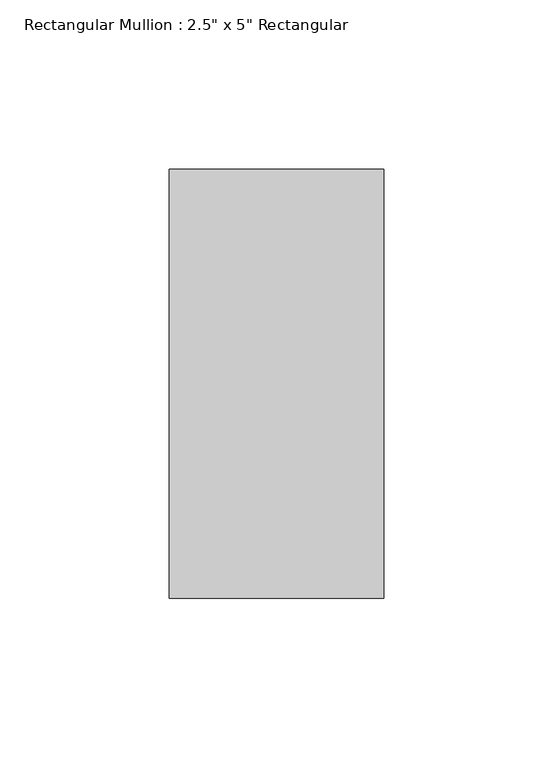
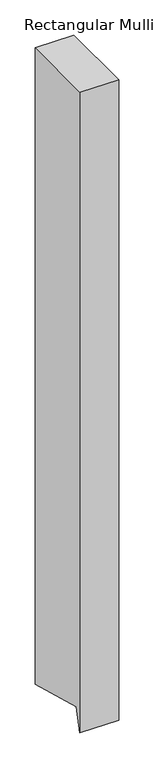
"""IFC4 building model written with IfcOpenShell, lengths in millimetres: member geometry."""

import ifcopenshell
import ifcopenshell.guid

model = None  # the IFC model being written
_history = None  # IfcOwnerHistory: only IFC2X3 demands one
_inside = {}  # id of a spatial element -> (the spatial element, [elements in it])
_under = {}  # id of a project, library or spatial element -> (it, [spatial elements below it])
_declared = {}  # id of a project -> (the project, [libraries it declares])
_typed = {}  # id of a type object -> (the type object, [elements of that type])
_made_of = {}  # id of a material, layer set ... -> (it, [elements and type objects made of it])


def new_model(schema):
    """Start an empty IFC model of exactly this schema.

    Asked for "IFC4X3", IfcOpenShell would pick the latest addendum, in which some entities
    have other attributes; the version numbers below select the first issue.
    IFC2X3 requires an IfcOwnerHistory on every rooted entity: one is made here for all.
    """
    global model, _history
    if schema == "IFC4X3":
        model = ifcopenshell.file(schema_version=(4, 3, 0, 0))
    else:
        model = ifcopenshell.file(schema=schema)
    _inside.clear()
    _under.clear()
    _declared.clear()
    _typed.clear()
    _made_of.clear()
    _history = None
    if model.schema == "IFC2X3":
        org = make("IfcOrganization", Name="unknown")
        user = make(
            "IfcPersonAndOrganization",
            ThePerson=make("IfcPerson", FamilyName="unknown"),
            TheOrganization=org,
        )
        app = make(
            "IfcApplication",
            ApplicationDeveloper=org,
            Version="unknown",
            ApplicationFullName="unknown",
            ApplicationIdentifier="unknown",
        )
        _history = make(
            "IfcOwnerHistory",
            OwningUser=user,
            OwningApplication=app,
            ChangeAction="ADDED",
            CreationDate=0,
        )
    return model


def make(cls, **values):
    """One entity of the class cls with the attributes given. An attribute that is None is left unset."""
    return model.create_entity(
        cls, **{name: value for name, value in values.items() if value is not None}
    )


def rooted(cls, **values):
    """An entity with a GlobalId (a new one), such as an element, a storey or a relation."""
    return make(cls, GlobalId=ifcopenshell.guid.new(), OwnerHistory=_history, **values)


def si_unit(unit_type, name, prefix=None):
    """IfcSIUnit, for example si_unit("LENGTHUNIT", "METRE", prefix="MILLI")."""
    return make("IfcSIUnit", UnitType=unit_type, Prefix=prefix, Name=name)


def assignment(units):
    """IfcUnitAssignment: the units of a project."""
    return None if units is None else make("IfcUnitAssignment", Units=units)


def point(xyz):
    """IfcCartesianPoint."""
    return None if xyz is None else make("IfcCartesianPoint", Coordinates=xyz)


def direction(xyz):
    """IfcDirection."""
    return None if xyz is None else make("IfcDirection", DirectionRatios=xyz)


def frame(location, z_axis=None, x_axis=None):
    """IfcAxis2Placement3D, a coordinate frame: its origin and axes. An axis left out is left unset."""
    return make(
        "IfcAxis2Placement3D",
        Location=point(location),
        Axis=direction(z_axis),
        RefDirection=direction(x_axis),
    )


def origin():
    """The frame at (0, 0, 0) with its axes left unset."""
    return frame((0.0, 0.0, 0.0))


def place(relative_to, where):
    """IfcLocalPlacement: puts the frame where relative to a parent placement (None: the world)."""
    return make(
        "IfcLocalPlacement", PlacementRelTo=relative_to, RelativePlacement=where
    )


def context(
    kind, dimensions, precision=None, world=None, true_north=None, identifier=None
):
    """IfcGeometricRepresentationContext, for example the 3D "Model" context."""
    return make(
        "IfcGeometricRepresentationContext",
        ContextIdentifier=identifier,
        ContextType=kind,
        CoordinateSpaceDimension=dimensions,
        Precision=precision,
        WorldCoordinateSystem=world,
        TrueNorth=true_north,
    )


def project(units=None, contexts=None):
    """IfcProject with its units and contexts."""
    return rooted(
        "IfcProject",
        Name="project",
        RepresentationContexts=contexts,
        UnitsInContext=assignment(units),
    )


def spatial(cls, under=None, at=None, **own):
    """A site, building, storey or space (cls), placed at a placement, below another one or the project."""
    s = rooted(cls, ObjectPlacement=at, **own)
    if under is not None:
        _under.setdefault(under.id(), (under, []))[1].append(s)
    return s


def polyline(points):
    """IfcPolyline through the points."""
    return make("IfcPolyline", Points=[point(p) for p in points])


def outline(outer, holes=None, kind="AREA"):
    """IfcArbitraryClosedProfileDef: a profile drawn as a closed curve; with holes, ...WithVoids."""
    if holes is None:
        return make("IfcArbitraryClosedProfileDef", ProfileType=kind, OuterCurve=outer)
    return make(
        "IfcArbitraryProfileDefWithVoids",
        ProfileType=kind,
        OuterCurve=outer,
        InnerCurves=holes,
    )


def extrude(swept, where, along, depth):
    """IfcExtrudedAreaSolid: the profile swept, set in the frame where, extruded along a direction by depth."""
    return make(
        "IfcExtrudedAreaSolid",
        SweptArea=swept,
        Position=where,
        ExtrudedDirection=direction(along),
        Depth=depth,
    )


def shape(context_of_items, identifier, shape_type, items):
    """IfcShapeRepresentation: the items that make up one representation, for example the "Body"."""
    return make(
        "IfcShapeRepresentation",
        ContextOfItems=context_of_items,
        RepresentationIdentifier=identifier,
        RepresentationType=shape_type,
        Items=items,
    )


def source(mapping_origin, context_of_items, identifier, shape_type, items):
    """IfcRepresentationMap: a shape defined once, which mapped items show again and again."""
    return make(
        "IfcRepresentationMap",
        MappingOrigin=mapping_origin,
        MappedRepresentation=shape(context_of_items, identifier, shape_type, items),
    )


def transform(
    local_origin,
    x_axis=None,
    y_axis=None,
    z_axis=None,
    scale=None,
    scale2=None,
    scale3=None,
    uniform=True,
):
    """IfcCartesianTransformationOperator3D, or its non-uniform kind. x_axis, y_axis, z_axis: its Axis1, 2, 3."""
    if uniform:
        return make(
            "IfcCartesianTransformationOperator3D",
            Axis1=direction(x_axis),
            Axis2=direction(y_axis),
            LocalOrigin=point(local_origin),
            Scale=scale,
            Axis3=direction(z_axis),
        )
    return make(
        "IfcCartesianTransformationOperator3DnonUniform",
        Axis1=direction(x_axis),
        Axis2=direction(y_axis),
        LocalOrigin=point(local_origin),
        Scale=scale,
        Axis3=direction(z_axis),
        Scale2=scale2,
        Scale3=scale3,
    )


def mapped(mapping_source, mapping_target):
    """IfcMappedItem: shows the shape of a source again, moved by a transform."""
    return make(
        "IfcMappedItem", MappingSource=mapping_source, MappingTarget=mapping_target
    )


def made_of(thing, what):
    """Note that an element or type object is made of a material, layer set ...; save() writes the relation."""
    if what is not None:
        _made_of.setdefault(what.id(), (what, []))[1].append(thing)
    return thing


def element(
    cls,
    number,
    at=None,
    inside=None,
    cuts=None,
    type_object=None,
    material=None,
    context=None,
    identifier="Body",
    shape_type=None,
    held_by="IfcProductDefinitionShape",
    body=None,
    shapes=None,
    **own,
):
    """One element of the class cls, such as IfcWall. Its Tag is "e" and its number.

    at: its placement. inside: the storey or other place that contains it. cuts: it is an
    opening in that element (IfcRelVoidsElement). A single representation is given by context,
    identifier, shape_type and body (its items); several are given by shapes. held_by: the class
    of the entity that holds the representations. save() writes the other relations.
    """
    e = rooted(cls, Tag="e%d" % number, ObjectPlacement=at, **own)
    if body is not None:
        shapes = [shape(context, identifier, shape_type, body)]
    if shapes is not None:
        e.Representation = make(held_by, Representations=shapes)
    if inside is not None:
        _inside.setdefault(inside.id(), (inside, []))[1].append(e)
    if cuts is not None:
        rooted(
            "IfcRelVoidsElement", RelatingBuildingElement=cuts, RelatedOpeningElement=e
        )
    if type_object is not None:
        _typed.setdefault(type_object.id(), (type_object, []))[1].append(e)
    return made_of(e, material)


def aggregate(whole, parts):
    """IfcRelAggregates: a whole, such as a stair, and the parts it consists of."""
    return rooted("IfcRelAggregates", RelatingObject=whole, RelatedObjects=parts)


def save(model, path):
    """Write the relations noted so far, then the file.

    IfcRelAggregates (storeys below a building ...), IfcRelContainedInSpatialStructure (elements
    in a storey), IfcRelDefinesByType, IfcRelAssociatesMaterial and IfcRelDeclares: one each for
    every whole, place, type object, material and project.
    """
    for whole, parts in _under.values():
        aggregate(whole, parts)
    for where, things in _inside.values():
        rooted(
            "IfcRelContainedInSpatialStructure",
            RelatedElements=things,
            RelatingStructure=where,
        )
    for kind, things in _typed.values():
        rooted("IfcRelDefinesByType", RelatedObjects=things, RelatingType=kind)
    for what, things in _made_of.values():
        rooted("IfcRelAssociatesMaterial", RelatedObjects=things, RelatingMaterial=what)
    for by, libraries in _declared.values():
        rooted("IfcRelDeclares", RelatingContext=by, RelatedDefinitions=libraries)
    model.write(path)


def member_0cfb68b1(model_context):
    return source(origin(), model_context, "Body", "SweptSolid", [
        extrude(outline(polyline([(-63.5, 0.0), (63.5, 0.0), (63.5, -1103.9654292), (-53.1187853, -1072.7175199), (-63.5, -1111.4607406), (-63.5, 0.0)])), frame((-63.5, 0.0, 0.0), z_axis=(1.0, 0.0, 0.0), x_axis=(0.0, 1.0, 0.0)), (0.0, 0.0, 1.0), 63.5),
    ])


if __name__ == "__main__":
    model = new_model("IFC4")
    model_context = context("Model", 3, world=origin())
    ifc_project = project(units=[si_unit("LENGTHUNIT", "METRE", prefix="MILLI")], contexts=[model_context])
    site = spatial("IfcSite", under=ifc_project)
    building = spatial("IfcBuilding", under=site)
    placement = place(None, origin())
    member_shape = member_0cfb68b1(model_context)
    element("IfcMember", 1, ObjectType="Rectangular Mullion : 2.5\" x 5\" Rectangular", at=placement, inside=building, context=model_context, shape_type="MappedRepresentation", body=[
        mapped(member_shape, transform((0.0, 0.0, 0.0), x_axis=(1.0, 0.0, 0.0), y_axis=(0.0, 1.0, 0.0), z_axis=(0.0, 0.0, 1.0))),
    ])
    save(model, "model.ifc")

# Revit data of these elements
# Type "Rectangular Mullion : 2.5\" x 5\" Rectangular"
#   built-in parameter 1007304 = 0.416667 (stored number, unit not read)
#   built-in parameter 1007301 = 0.104167 (stored number, unit not read)
#   built-in parameter 1007300 = 0.104167 (stored number, unit not read)
# Element 1 (IfcMember, "Rectangular Mullion : 2.5\" x 5\" Rectangular")
#   Materials on its faces: "Aluminum"
# Materials
#   "Aluminum": class "Metal", colour RGB 247 247 247, transparency 0, Description = "Aluminum 6061", Cost = 0
